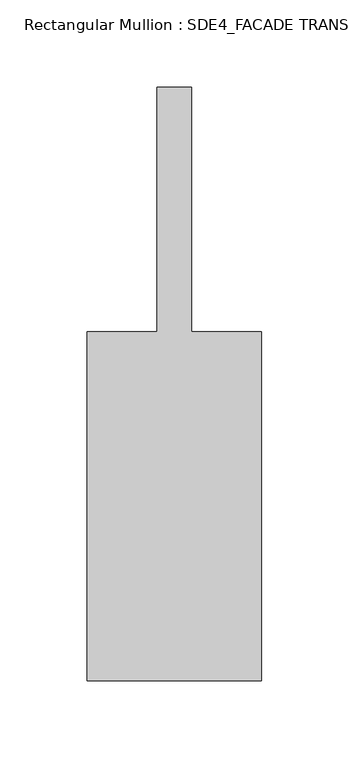
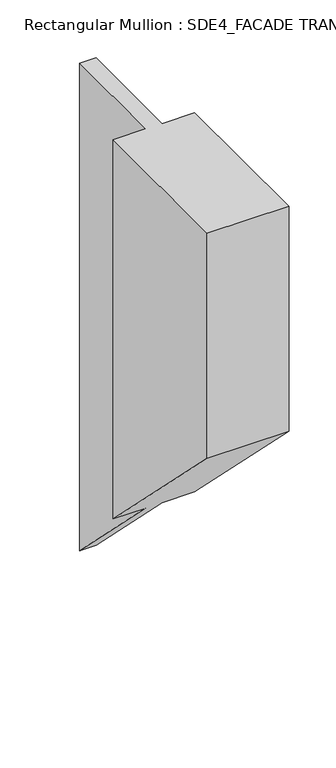
"""IFC4 building model written with IfcOpenShell, lengths in millimetres: member geometry, Rectangular Mullion : SDE4_FACADE TRANSOM TYPE 1."""

from ifc_helpers import new_model, si_unit, origin, place, context, project, spatial, faceted_brep, source, transform, mapped, element, save


def rectangular_mullion_sde4_facade_transom_type_1_5e3b8767(model_context):
    return source(origin(), model_context, "Body", "Brep", [
        faceted_brep([(50.0, -132.5, 0.0), (50.0, 67.5, 0.0), (10.0, 67.5, 0.0), (10.0, 207.5, 0.0), (-10.0, 207.5, 0.0), (-10.0, 67.5, 0.0), (-50.0, 67.5, 0.0), (-50.0, -132.5, 0.0), (50.0, -132.5, -290.7805066), (50.0, 67.5, -490.7805066), (10.0, 67.5, -490.7805066), (10.0, 207.5, -630.7805066), (-10.0, 207.5, -630.7805066), (-10.0, 67.5, -490.7805066), (-50.0, 67.5, -490.7805066), (-50.0, -132.5, -290.7805066)], [[[0, 1, 2, 3, 4, 5, 6, 7]], [[1, 0, 8, 9]], [[2, 1, 9, 10]], [[3, 2, 10, 11]], [[4, 3, 11, 12]], [[5, 4, 12, 13]], [[6, 5, 13, 14]], [[7, 6, 14, 15]], [[0, 7, 15, 8]], [[8, 15, 14, 13, 12, 11, 10, 9]]]),
    ])


if __name__ == "__main__":
    model = new_model("IFC4")
    model_context = context("Model", 3, world=origin())
    ifc_project = project(units=[si_unit("LENGTHUNIT", "METRE", prefix="MILLI")], contexts=[model_context])
    site = spatial("IfcSite", under=ifc_project)
    building = spatial("IfcBuilding", under=site)
    placement = place(None, origin())
    rectangular_mullion_sde4_facade_transom_type_1_shape = rectangular_mullion_sde4_facade_transom_type_1_5e3b8767(model_context)
    element("IfcMember", 1, ObjectType="Rectangular Mullion : SDE4_FACADE TRANSOM TYPE 1", at=placement, inside=building, context=model_context, shape_type="MappedRepresentation", body=[
        mapped(rectangular_mullion_sde4_facade_transom_type_1_shape, transform((0.0, 0.0, 0.0), x_axis=(1.0, 0.0, 0.0), y_axis=(0.0, 1.0, 0.0), z_axis=(0.0, 0.0, 1.0))),
    ])
    save(model, "model.ifc")

# Revit data of these elements
# Type "Rectangular Mullion : SDE4_FACADE TRANSOM TYPE 1"
#   built-in parameter 1007322 = 1.11549 (stored number, unit not read)
#   built-in parameter 1007321 = 0.164042 (stored number, unit not read)
#   built-in parameter 1007320 = 0.164042 (stored number, unit not read)
